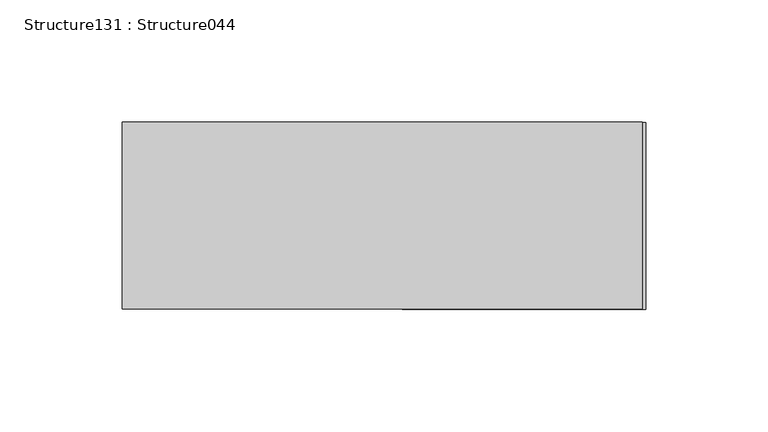
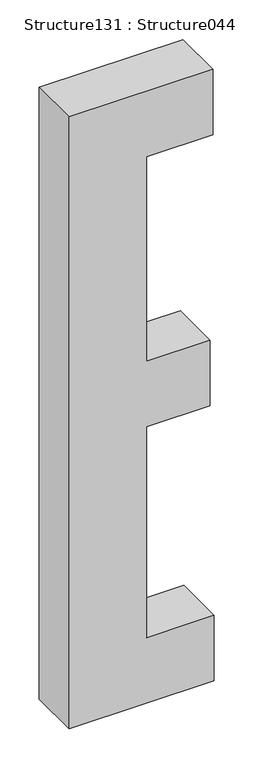
"""IFC4 building model written with IfcOpenShell, lengths in millimetres: proxy geometry, Structure131 : Structure044."""

from ifc_helpers import new_model, si_unit, frame, origin, place, context, project, spatial, polyline, outline, extrude, source, transform, mapped, element, save


def structure131_structure044_92eb0eea(model_context):
    return source(origin(), model_context, "Body", "SweptSolid", [
        extrude(outline(polyline([(4480.4419946, -46896.8615358), (3528.5825142, -46896.8615358), (3528.5825142, -46683.3731162), (3630.5630275, -46683.3731162), (3630.5630275, -46782.6253993), (3958.2800261, -46782.6253993), (3958.2800261, -46688.8138319), (4060.2611693, -46688.8138319), (4060.2611693, -46782.6253993), (4378.4602217, -46782.6253993), (4378.4602217, -46684.7290441), (4480.4419946, -46684.7290441), (4480.4419946, -46896.8615358)])), frame((0.0, 247945.1599557, 0.0), z_axis=(0.0, 1.0, 0.0), x_axis=(0.0, 0.0, 1.0)), (0.0, 0.0, 1.0), 76.2),
    ])


if __name__ == "__main__":
    model = new_model("IFC4")
    model_context = context("Model", 3, world=origin())
    ifc_project = project(units=[si_unit("LENGTHUNIT", "METRE", prefix="MILLI")], contexts=[model_context])
    site = spatial("IfcSite", under=ifc_project)
    building = spatial("IfcBuilding", under=site)
    placement = place(None, origin())
    structure131_structure044_shape = structure131_structure044_92eb0eea(model_context)
    element("IfcBuildingElementProxy", 1, Name="Structure131 : Structure044", ObjectType="Structure131 : Structure044", at=placement, inside=building, context=model_context, shape_type="MappedRepresentation", body=[
        mapped(structure131_structure044_shape, transform((0.0, 0.0, 0.0), x_axis=(1.0, 0.0, 0.0), y_axis=(0.0, 1.0, 0.0), z_axis=(0.0, 0.0, 1.0))),
    ])
    save(model, "model.ifc")

# Revit data of these elements
# Type "Structure131 : Structure044"
#   NameOverride = "Structure044"
# Element 1 (IfcBuildingElementProxy, "Structure131 : Structure044")
#   Materials on its faces: "BRUSHED ALUM. LETTERING"
# Materials
#   "BRUSHED ALUM. LETTERING": class "Unassigned", colour RGB 169 181 186, transparency 0, Cost = 0
